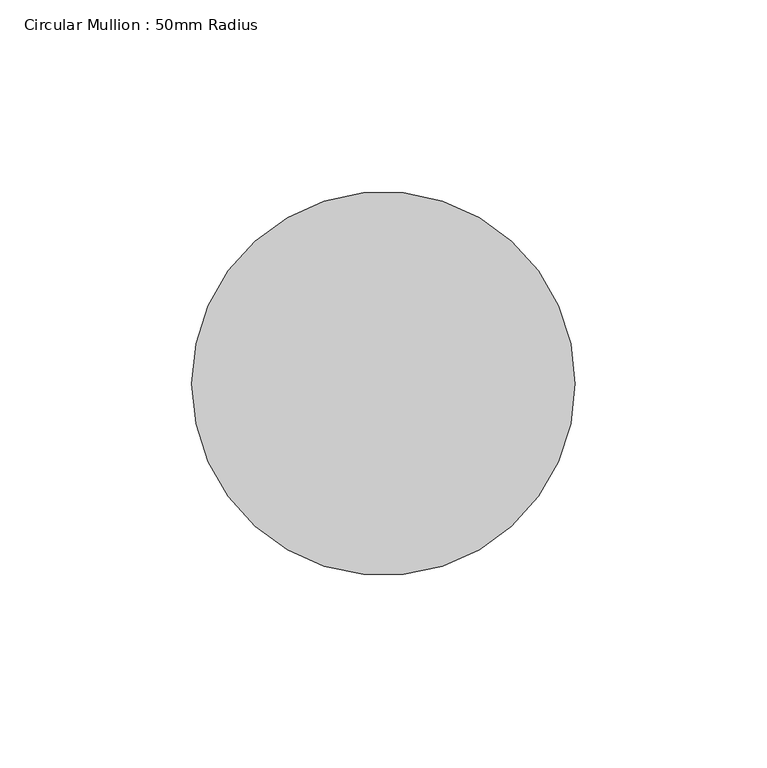
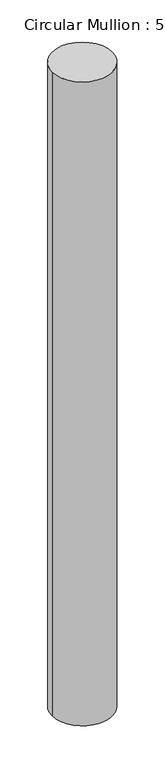
"""IFC4 building model written with IfcOpenShell, lengths in millimetres: member geometry, Circular Mullion : 50mm Radius."""

import ifcopenshell
import ifcopenshell.guid

model = None  # the IFC model being written
_history = None  # IfcOwnerHistory: only IFC2X3 demands one
_inside = {}  # id of a spatial element -> (the spatial element, [elements in it])
_under = {}  # id of a project, library or spatial element -> (it, [spatial elements below it])
_declared = {}  # id of a project -> (the project, [libraries it declares])
_typed = {}  # id of a type object -> (the type object, [elements of that type])
_made_of = {}  # id of a material, layer set ... -> (it, [elements and type objects made of it])


def new_model(schema):
    """Start an empty IFC model of exactly this schema.

    Asked for "IFC4X3", IfcOpenShell would pick the latest addendum, in which some entities
    have other attributes; the version numbers below select the first issue.
    IFC2X3 requires an IfcOwnerHistory on every rooted entity: one is made here for all.
    """
    global model, _history
    if schema == "IFC4X3":
        model = ifcopenshell.file(schema_version=(4, 3, 0, 0))
    else:
        model = ifcopenshell.file(schema=schema)
    _inside.clear()
    _under.clear()
    _declared.clear()
    _typed.clear()
    _made_of.clear()
    _history = None
    if model.schema == "IFC2X3":
        org = make("IfcOrganization", Name="unknown")
        user = make(
            "IfcPersonAndOrganization",
            ThePerson=make("IfcPerson", FamilyName="unknown"),
            TheOrganization=org,
        )
        app = make(
            "IfcApplication",
            ApplicationDeveloper=org,
            Version="unknown",
            ApplicationFullName="unknown",
            ApplicationIdentifier="unknown",
        )
        _history = make(
            "IfcOwnerHistory",
            OwningUser=user,
            OwningApplication=app,
            ChangeAction="ADDED",
            CreationDate=0,
        )
    return model


def make(cls, **values):
    """One entity of the class cls with the attributes given. An attribute that is None is left unset."""
    return model.create_entity(
        cls, **{name: value for name, value in values.items() if value is not None}
    )


def rooted(cls, **values):
    """An entity with a GlobalId (a new one), such as an element, a storey or a relation."""
    return make(cls, GlobalId=ifcopenshell.guid.new(), OwnerHistory=_history, **values)


def si_unit(unit_type, name, prefix=None):
    """IfcSIUnit, for example si_unit("LENGTHUNIT", "METRE", prefix="MILLI")."""
    return make("IfcSIUnit", UnitType=unit_type, Prefix=prefix, Name=name)


def assignment(units):
    """IfcUnitAssignment: the units of a project."""
    return None if units is None else make("IfcUnitAssignment", Units=units)


def point(xyz):
    """IfcCartesianPoint."""
    return None if xyz is None else make("IfcCartesianPoint", Coordinates=xyz)


def direction(xyz):
    """IfcDirection."""
    return None if xyz is None else make("IfcDirection", DirectionRatios=xyz)


def frame(location, z_axis=None, x_axis=None):
    """IfcAxis2Placement3D, a coordinate frame: its origin and axes. An axis left out is left unset."""
    return make(
        "IfcAxis2Placement3D",
        Location=point(location),
        Axis=direction(z_axis),
        RefDirection=direction(x_axis),
    )


def frame_2d(location, x_axis=None):
    """IfcAxis2Placement2D, a coordinate frame in the plane: its origin and x axis."""
    return make(
        "IfcAxis2Placement2D", Location=point(location), RefDirection=direction(x_axis)
    )


def origin():
    """The frame at (0, 0, 0) with its axes left unset."""
    return frame((0.0, 0.0, 0.0))


def origin_2d():
    """The frame at (0, 0) in the plane with its x axis left unset."""
    return frame_2d((0.0, 0.0))


def place(relative_to, where):
    """IfcLocalPlacement: puts the frame where relative to a parent placement (None: the world)."""
    return make(
        "IfcLocalPlacement", PlacementRelTo=relative_to, RelativePlacement=where
    )


def context(
    kind, dimensions, precision=None, world=None, true_north=None, identifier=None
):
    """IfcGeometricRepresentationContext, for example the 3D "Model" context."""
    return make(
        "IfcGeometricRepresentationContext",
        ContextIdentifier=identifier,
        ContextType=kind,
        CoordinateSpaceDimension=dimensions,
        Precision=precision,
        WorldCoordinateSystem=world,
        TrueNorth=true_north,
    )


def project(units=None, contexts=None):
    """IfcProject with its units and contexts."""
    return rooted(
        "IfcProject",
        Name="project",
        RepresentationContexts=contexts,
        UnitsInContext=assignment(units),
    )


def spatial(cls, under=None, at=None, **own):
    """A site, building, storey or space (cls), placed at a placement, below another one or the project."""
    s = rooted(cls, ObjectPlacement=at, **own)
    if under is not None:
        _under.setdefault(under.id(), (under, []))[1].append(s)
    return s


def circle_curve(where, radius):
    """IfcCircle in the frame where."""
    return make("IfcCircle", Position=where, Radius=radius)


def trimmed(basis, trim1, trim2, sense, master):
    """IfcTrimmedCurve: the piece of a basis curve between two trims."""
    return make(
        "IfcTrimmedCurve",
        BasisCurve=basis,
        Trim1=trim1,
        Trim2=trim2,
        SenseAgreement=sense,
        MasterRepresentation=master,
    )


def segment(curve, same_sense, transition):
    """IfcCompositeCurveSegment."""
    return make(
        "IfcCompositeCurveSegment",
        Transition=transition,
        SameSense=same_sense,
        ParentCurve=curve,
    )


def composite_curve(segments, self_intersect=None):
    """IfcCompositeCurve: segments joined end to end."""
    return make("IfcCompositeCurve", Segments=segments, SelfIntersect=self_intersect)


def outline(outer, holes=None, kind="AREA"):
    """IfcArbitraryClosedProfileDef: a profile drawn as a closed curve; with holes, ...WithVoids."""
    if holes is None:
        return make("IfcArbitraryClosedProfileDef", ProfileType=kind, OuterCurve=outer)
    return make(
        "IfcArbitraryProfileDefWithVoids",
        ProfileType=kind,
        OuterCurve=outer,
        InnerCurves=holes,
    )


def extrude(swept, where, along, depth):
    """IfcExtrudedAreaSolid: the profile swept, set in the frame where, extruded along a direction by depth."""
    return make(
        "IfcExtrudedAreaSolid",
        SweptArea=swept,
        Position=where,
        ExtrudedDirection=direction(along),
        Depth=depth,
    )


def shape(context_of_items, identifier, shape_type, items):
    """IfcShapeRepresentation: the items that make up one representation, for example the "Body"."""
    return make(
        "IfcShapeRepresentation",
        ContextOfItems=context_of_items,
        RepresentationIdentifier=identifier,
        RepresentationType=shape_type,
        Items=items,
    )


def source(mapping_origin, context_of_items, identifier, shape_type, items):
    """IfcRepresentationMap: a shape defined once, which mapped items show again and again."""
    return make(
        "IfcRepresentationMap",
        MappingOrigin=mapping_origin,
        MappedRepresentation=shape(context_of_items, identifier, shape_type, items),
    )


def transform(
    local_origin,
    x_axis=None,
    y_axis=None,
    z_axis=None,
    scale=None,
    scale2=None,
    scale3=None,
    uniform=True,
):
    """IfcCartesianTransformationOperator3D, or its non-uniform kind. x_axis, y_axis, z_axis: its Axis1, 2, 3."""
    if uniform:
        return make(
            "IfcCartesianTransformationOperator3D",
            Axis1=direction(x_axis),
            Axis2=direction(y_axis),
            LocalOrigin=point(local_origin),
            Scale=scale,
            Axis3=direction(z_axis),
        )
    return make(
        "IfcCartesianTransformationOperator3DnonUniform",
        Axis1=direction(x_axis),
        Axis2=direction(y_axis),
        LocalOrigin=point(local_origin),
        Scale=scale,
        Axis3=direction(z_axis),
        Scale2=scale2,
        Scale3=scale3,
    )


def mapped(mapping_source, mapping_target):
    """IfcMappedItem: shows the shape of a source again, moved by a transform."""
    return make(
        "IfcMappedItem", MappingSource=mapping_source, MappingTarget=mapping_target
    )


def made_of(thing, what):
    """Note that an element or type object is made of a material, layer set ...; save() writes the relation."""
    if what is not None:
        _made_of.setdefault(what.id(), (what, []))[1].append(thing)
    return thing


def element(
    cls,
    number,
    at=None,
    inside=None,
    cuts=None,
    type_object=None,
    material=None,
    context=None,
    identifier="Body",
    shape_type=None,
    held_by="IfcProductDefinitionShape",
    body=None,
    shapes=None,
    **own,
):
    """One element of the class cls, such as IfcWall. Its Tag is "e" and its number.

    at: its placement. inside: the storey or other place that contains it. cuts: it is an
    opening in that element (IfcRelVoidsElement). A single representation is given by context,
    identifier, shape_type and body (its items); several are given by shapes. held_by: the class
    of the entity that holds the representations. save() writes the other relations.
    """
    e = rooted(cls, Tag="e%d" % number, ObjectPlacement=at, **own)
    if body is not None:
        shapes = [shape(context, identifier, shape_type, body)]
    if shapes is not None:
        e.Representation = make(held_by, Representations=shapes)
    if inside is not None:
        _inside.setdefault(inside.id(), (inside, []))[1].append(e)
    if cuts is not None:
        rooted(
            "IfcRelVoidsElement", RelatingBuildingElement=cuts, RelatedOpeningElement=e
        )
    if type_object is not None:
        _typed.setdefault(type_object.id(), (type_object, []))[1].append(e)
    return made_of(e, material)


def aggregate(whole, parts):
    """IfcRelAggregates: a whole, such as a stair, and the parts it consists of."""
    return rooted("IfcRelAggregates", RelatingObject=whole, RelatedObjects=parts)


def save(model, path):
    """Write the relations noted so far, then the file.

    IfcRelAggregates (storeys below a building ...), IfcRelContainedInSpatialStructure (elements
    in a storey), IfcRelDefinesByType, IfcRelAssociatesMaterial and IfcRelDeclares: one each for
    every whole, place, type object, material and project.
    """
    for whole, parts in _under.values():
        aggregate(whole, parts)
    for where, things in _inside.values():
        rooted(
            "IfcRelContainedInSpatialStructure",
            RelatedElements=things,
            RelatingStructure=where,
        )
    for kind, things in _typed.values():
        rooted("IfcRelDefinesByType", RelatedObjects=things, RelatingType=kind)
    for what, things in _made_of.values():
        rooted("IfcRelAssociatesMaterial", RelatedObjects=things, RelatingMaterial=what)
    for by, libraries in _declared.values():
        rooted("IfcRelDeclares", RelatingContext=by, RelatedDefinitions=libraries)
    model.write(path)


def circular_mullion_50mm_radius_226fc1f1(model_context):
    return source(origin(), model_context, "Body", "SweptSolid", [
        extrude(outline(composite_curve([segment(trimmed(circle_curve(origin_2d(), 50.0), [point((50.0, 0.0))], [point((-50.0, 0.0))], False, "CARTESIAN"), True, "CONTINUOUS"), segment(trimmed(circle_curve(origin_2d(), 50.0), [point((-50.0, 0.0))], [point((50.0, 0.0))], False, "CARTESIAN"), True, "CONTINUOUS")], self_intersect=False)), frame((0.0, 0.0, -1133.5689179), z_axis=(0.0, 0.0, 1.0), x_axis=(1.0, 0.0, 0.0)), (0.0, 0.0, 1.0), 1133.5689179),
    ])


if __name__ == "__main__":
    model = new_model("IFC4")
    model_context = context("Model", 3, world=origin())
    ifc_project = project(units=[si_unit("LENGTHUNIT", "METRE", prefix="MILLI")], contexts=[model_context])
    site = spatial("IfcSite", under=ifc_project)
    building = spatial("IfcBuilding", under=site)
    placement = place(None, origin())
    circular_mullion_50mm_radius_shape = circular_mullion_50mm_radius_226fc1f1(model_context)
    element("IfcMember", 1, ObjectType="Circular Mullion : 50mm Radius", at=placement, inside=building, context=model_context, shape_type="MappedRepresentation", body=[
        mapped(circular_mullion_50mm_radius_shape, transform((0.0, 0.0, 0.0), x_axis=(1.0, 0.0, 0.0), y_axis=(0.0, 1.0, 0.0), z_axis=(0.0, 0.0, 1.0))),
    ])
    save(model, "model.ifc")

# Revit data of these elements
# Type "Circular Mullion : 50mm Radius"
#   built-in parameter 1007350 = 0.164042 (stored number, unit not read)
# Element 1 (IfcMember, "Circular Mullion : 50mm Radius")
#   Materials on its faces: "Aluminium"
# Materials
#   "Aluminium": class "Metal", colour RGB 247 247 247, transparency 0, Description = "Aluminium 6061", Cost = 0
